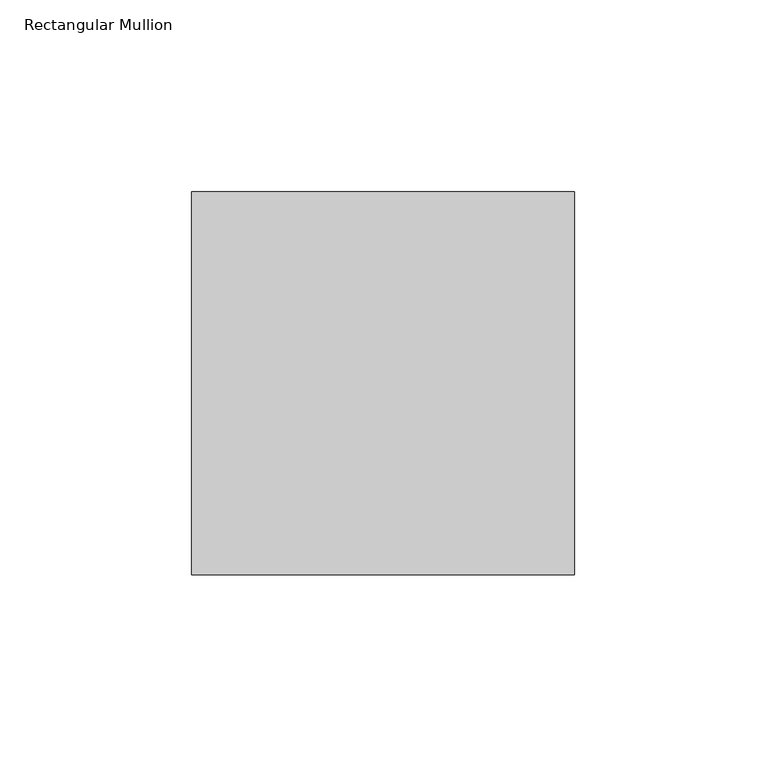
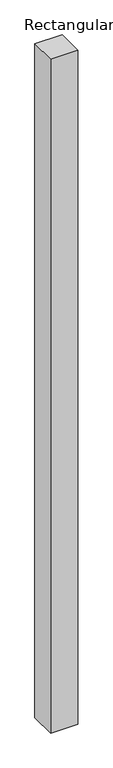
"""IFC4 building model written with IfcOpenShell, lengths in millimetres: member geometry, Rectangular Mullion : 알루미늄_Rectangular Cap_100 x100."""

from ifc_helpers import new_model, si_unit, frame, origin, place, context, project, spatial, polyline, outline, extrude, source, transform, mapped, element, save


def rectangular_mullion_2343147e(model_context):
    return source(origin(), model_context, "Body", "SweptSolid", [
        extrude(outline(polyline([(0.0, 50.0), (0.0, -50.0), (-100.0, -50.0), (-100.0, 50.0), (0.0, 50.0)])), frame((0.0, 0.0, -2625.0), z_axis=(0.0, 0.0, 1.0), x_axis=(1.0, 0.0, 0.0)), (0.0, 0.0, 1.0), 2625.0),
    ])


if __name__ == "__main__":
    model = new_model("IFC4")
    model_context = context("Model", 3, world=origin())
    ifc_project = project(units=[si_unit("LENGTHUNIT", "METRE", prefix="MILLI")], contexts=[model_context])
    site = spatial("IfcSite", under=ifc_project)
    building = spatial("IfcBuilding", under=site)
    placement = place(None, origin())
    rectangular_mullion_shape = rectangular_mullion_2343147e(model_context)
    element("IfcMember", 1, ObjectType="Rectangular Mullion : 알루미늄_Rectangular Cap_100 x100", at=placement, inside=building, context=model_context, shape_type="MappedRepresentation", body=[
        mapped(rectangular_mullion_shape, transform((0.0, 0.0, 0.0), x_axis=(1.0, 0.0, 0.0), y_axis=(0.0, 1.0, 0.0), z_axis=(0.0, 0.0, 1.0))),
    ])
    save(model, "model.ifc")

# Revit data of these elements
# Type "Rectangular Mullion : 알루미늄_Rectangular Cap_100 x100"
#   built-in parameter 1007304 = 0.328084 (stored number, unit not read)
#   built-in parameter 1007301 = 0.164042 (stored number, unit not read)
#   built-in parameter 1007300 = 0.164042 (stored number, unit not read)
# Element 1 (IfcMember, "Rectangular Mullion : 알루미늄_Rectangular Cap_100 x100")
#   Materials on its faces: "00_Metal_Stainless Steel"
# Materials
#   "00_Metal_Stainless Steel": class "Metal", colour RGB 148 148 148, transparency 0, Description = "Steel", Cost = 0
